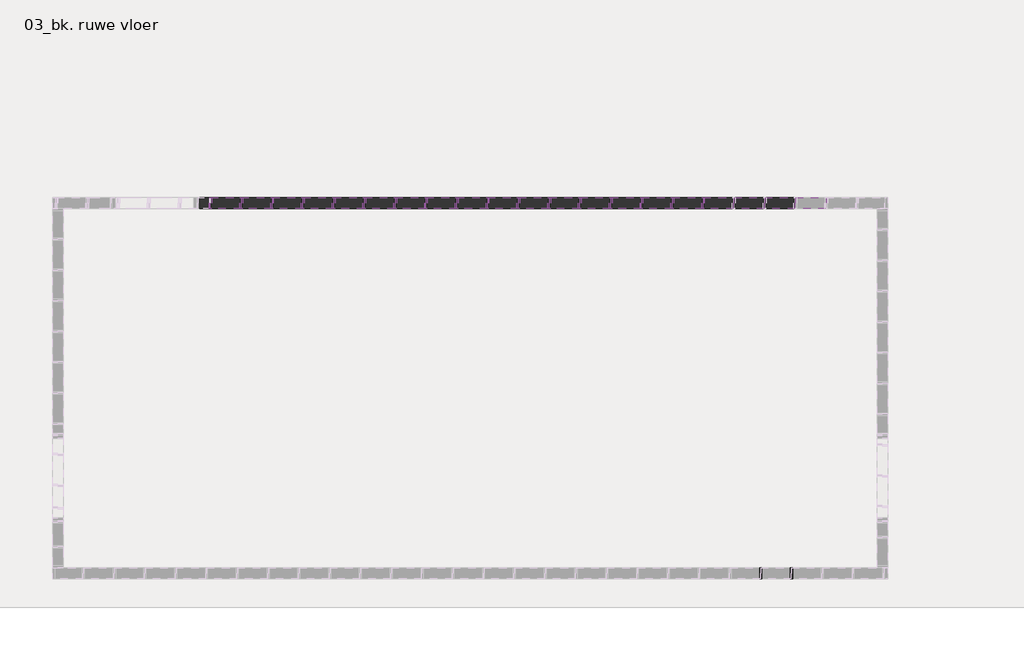
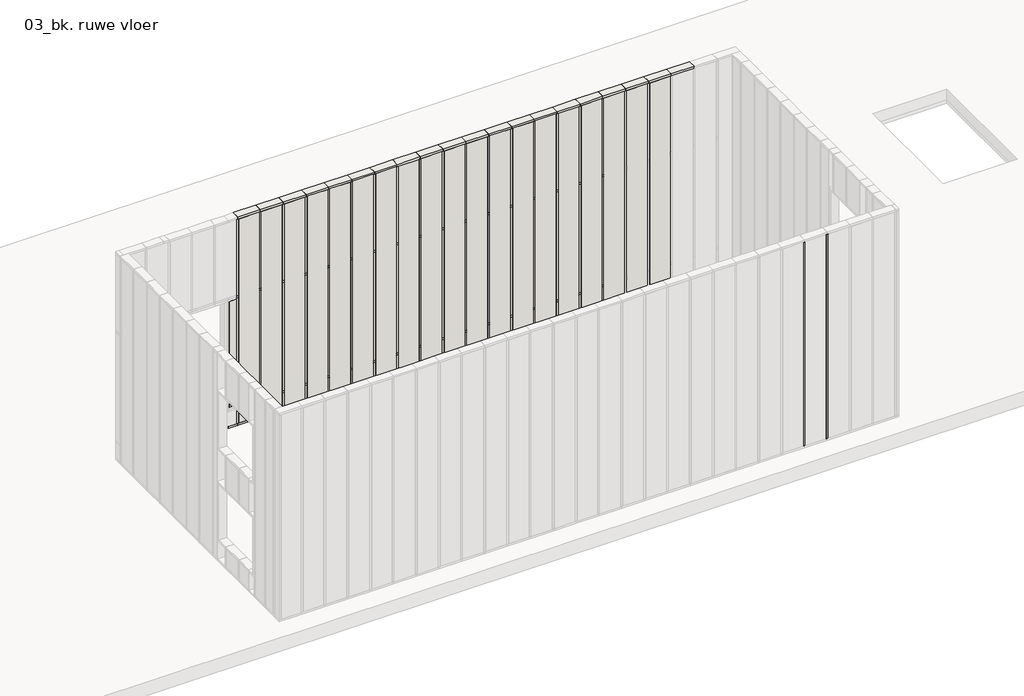
# One storey, part 3 of 9: 144 walls.
"""IFC4 building model written with IfcOpenShell, lengths in millimetres."""

import ifcopenshell
import ifcopenshell.guid

model = None  # the IFC model being written
_history = None  # IfcOwnerHistory: only IFC2X3 demands one
_inside = {}  # id of a spatial element -> (the spatial element, [elements in it])
_under = {}  # id of a project, library or spatial element -> (it, [spatial elements below it])
_declared = {}  # id of a project -> (the project, [libraries it declares])
_typed = {}  # id of a type object -> (the type object, [elements of that type])
_made_of = {}  # id of a material, layer set ... -> (it, [elements and type objects made of it])


def new_model(schema):
    """Start an empty IFC model of exactly this schema.

    Asked for "IFC4X3", IfcOpenShell would pick the latest addendum, in which some entities
    have other attributes; the version numbers below select the first issue.
    IFC2X3 requires an IfcOwnerHistory on every rooted entity: one is made here for all.
    """
    global model, _history
    if schema == "IFC4X3":
        model = ifcopenshell.file(schema_version=(4, 3, 0, 0))
    else:
        model = ifcopenshell.file(schema=schema)
    _inside.clear()
    _under.clear()
    _declared.clear()
    _typed.clear()
    _made_of.clear()
    _history = None
    if model.schema == "IFC2X3":
        org = make("IfcOrganization", Name="unknown")
        user = make(
            "IfcPersonAndOrganization",
            ThePerson=make("IfcPerson", FamilyName="unknown"),
            TheOrganization=org,
        )
        app = make(
            "IfcApplication",
            ApplicationDeveloper=org,
            Version="unknown",
            ApplicationFullName="unknown",
            ApplicationIdentifier="unknown",
        )
        _history = make(
            "IfcOwnerHistory",
            OwningUser=user,
            OwningApplication=app,
            ChangeAction="ADDED",
            CreationDate=0,
        )
    return model


def make(cls, **values):
    """One entity of the class cls with the attributes given. An attribute that is None is left unset."""
    return model.create_entity(
        cls, **{name: value for name, value in values.items() if value is not None}
    )


def rooted(cls, **values):
    """An entity with a GlobalId (a new one), such as an element, a storey or a relation."""
    return make(cls, GlobalId=ifcopenshell.guid.new(), OwnerHistory=_history, **values)


def si_unit(unit_type, name, prefix=None):
    """IfcSIUnit, for example si_unit("LENGTHUNIT", "METRE", prefix="MILLI")."""
    return make("IfcSIUnit", UnitType=unit_type, Prefix=prefix, Name=name)


def assignment(units):
    """IfcUnitAssignment: the units of a project."""
    return None if units is None else make("IfcUnitAssignment", Units=units)


def point(xyz):
    """IfcCartesianPoint."""
    return None if xyz is None else make("IfcCartesianPoint", Coordinates=xyz)


def direction(xyz):
    """IfcDirection."""
    return None if xyz is None else make("IfcDirection", DirectionRatios=xyz)


def frame(location, z_axis=None, x_axis=None):
    """IfcAxis2Placement3D, a coordinate frame: its origin and axes. An axis left out is left unset."""
    return make(
        "IfcAxis2Placement3D",
        Location=point(location),
        Axis=direction(z_axis),
        RefDirection=direction(x_axis),
    )


def origin():
    """The frame at (0, 0, 0) with its axes left unset."""
    return frame((0.0, 0.0, 0.0))


def origin_with_axes():
    """The frame at (0, 0, 0) with the z axis (0, 0, 1) and the x axis (1, 0, 0) written out."""
    return frame((0.0, 0.0, 0.0), z_axis=(0.0, 0.0, 1.0), x_axis=(1.0, 0.0, 0.0))


def place(relative_to, where):
    """IfcLocalPlacement: puts the frame where relative to a parent placement (None: the world)."""
    return make(
        "IfcLocalPlacement", PlacementRelTo=relative_to, RelativePlacement=where
    )


def context(
    kind, dimensions, precision=None, world=None, true_north=None, identifier=None
):
    """IfcGeometricRepresentationContext, for example the 3D "Model" context."""
    return make(
        "IfcGeometricRepresentationContext",
        ContextIdentifier=identifier,
        ContextType=kind,
        CoordinateSpaceDimension=dimensions,
        Precision=precision,
        WorldCoordinateSystem=world,
        TrueNorth=true_north,
    )


def project(units=None, contexts=None):
    """IfcProject with its units and contexts."""
    return rooted(
        "IfcProject",
        Name="project",
        RepresentationContexts=contexts,
        UnitsInContext=assignment(units),
    )


def spatial(cls, under=None, at=None, **own):
    """A site, building, storey or space (cls), placed at a placement, below another one or the project."""
    s = rooted(cls, ObjectPlacement=at, **own)
    if under is not None:
        _under.setdefault(under.id(), (under, []))[1].append(s)
    return s


def polyline(points):
    """IfcPolyline through the points."""
    return make("IfcPolyline", Points=[point(p) for p in points])


def outline(outer, holes=None, kind="AREA"):
    """IfcArbitraryClosedProfileDef: a profile drawn as a closed curve; with holes, ...WithVoids."""
    if holes is None:
        return make("IfcArbitraryClosedProfileDef", ProfileType=kind, OuterCurve=outer)
    return make(
        "IfcArbitraryProfileDefWithVoids",
        ProfileType=kind,
        OuterCurve=outer,
        InnerCurves=holes,
    )


def extrude(swept, where, along, depth):
    """IfcExtrudedAreaSolid: the profile swept, set in the frame where, extruded along a direction by depth."""
    return make(
        "IfcExtrudedAreaSolid",
        SweptArea=swept,
        Position=where,
        ExtrudedDirection=direction(along),
        Depth=depth,
    )


def shape(context_of_items, identifier, shape_type, items):
    """IfcShapeRepresentation: the items that make up one representation, for example the "Body"."""
    return make(
        "IfcShapeRepresentation",
        ContextOfItems=context_of_items,
        RepresentationIdentifier=identifier,
        RepresentationType=shape_type,
        Items=items,
    )


def source(mapping_origin, context_of_items, identifier, shape_type, items):
    """IfcRepresentationMap: a shape defined once, which mapped items show again and again."""
    return make(
        "IfcRepresentationMap",
        MappingOrigin=mapping_origin,
        MappedRepresentation=shape(context_of_items, identifier, shape_type, items),
    )


def transform(
    local_origin,
    x_axis=None,
    y_axis=None,
    z_axis=None,
    scale=None,
    scale2=None,
    scale3=None,
    uniform=True,
):
    """IfcCartesianTransformationOperator3D, or its non-uniform kind. x_axis, y_axis, z_axis: its Axis1, 2, 3."""
    if uniform:
        return make(
            "IfcCartesianTransformationOperator3D",
            Axis1=direction(x_axis),
            Axis2=direction(y_axis),
            LocalOrigin=point(local_origin),
            Scale=scale,
            Axis3=direction(z_axis),
        )
    return make(
        "IfcCartesianTransformationOperator3DnonUniform",
        Axis1=direction(x_axis),
        Axis2=direction(y_axis),
        LocalOrigin=point(local_origin),
        Scale=scale,
        Axis3=direction(z_axis),
        Scale2=scale2,
        Scale3=scale3,
    )


def mapped(mapping_source, mapping_target):
    """IfcMappedItem: shows the shape of a source again, moved by a transform."""
    return make(
        "IfcMappedItem", MappingSource=mapping_source, MappingTarget=mapping_target
    )


def made_of(thing, what):
    """Note that an element or type object is made of a material, layer set ...; save() writes the relation."""
    if what is not None:
        _made_of.setdefault(what.id(), (what, []))[1].append(thing)
    return thing


def element(
    cls,
    number,
    at=None,
    inside=None,
    cuts=None,
    type_object=None,
    material=None,
    context=None,
    identifier="Body",
    shape_type=None,
    held_by="IfcProductDefinitionShape",
    body=None,
    shapes=None,
    **own,
):
    """One element of the class cls, such as IfcWall. Its Tag is "e" and its number.

    at: its placement. inside: the storey or other place that contains it. cuts: it is an
    opening in that element (IfcRelVoidsElement). A single representation is given by context,
    identifier, shape_type and body (its items); several are given by shapes. held_by: the class
    of the entity that holds the representations. save() writes the other relations.
    """
    e = rooted(cls, Tag="e%d" % number, ObjectPlacement=at, **own)
    if body is not None:
        shapes = [shape(context, identifier, shape_type, body)]
    if shapes is not None:
        e.Representation = make(held_by, Representations=shapes)
    if inside is not None:
        _inside.setdefault(inside.id(), (inside, []))[1].append(e)
    if cuts is not None:
        rooted(
            "IfcRelVoidsElement", RelatingBuildingElement=cuts, RelatedOpeningElement=e
        )
    if type_object is not None:
        _typed.setdefault(type_object.id(), (type_object, []))[1].append(e)
    return made_of(e, material)


def aggregate(whole, parts):
    """IfcRelAggregates: a whole, such as a stair, and the parts it consists of."""
    return rooted("IfcRelAggregates", RelatingObject=whole, RelatedObjects=parts)


def save(model, path):
    """Write the relations noted so far, then the file.

    IfcRelAggregates (storeys below a building ...), IfcRelContainedInSpatialStructure (elements
    in a storey), IfcRelDefinesByType, IfcRelAssociatesMaterial and IfcRelDeclares: one each for
    every whole, place, type object, material and project.
    """
    for whole, parts in _under.values():
        aggregate(whole, parts)
    for where, things in _inside.values():
        rooted(
            "IfcRelContainedInSpatialStructure",
            RelatedElements=things,
            RelatingStructure=where,
        )
    for kind, things in _typed.values():
        rooted("IfcRelDefinesByType", RelatedObjects=things, RelatingType=kind)
    for what, things in _made_of.values():
        rooted("IfcRelAssociatesMaterial", RelatedObjects=things, RelatingMaterial=what)
    for by, libraries in _declared.values():
        rooted("IfcRelDeclares", RelatingContext=by, RelatedDefinitions=libraries)
    model.write(path)


def rectangular_mullion_51268c3e(model_context):
    return source(origin(), model_context, "Body", "SweptSolid", [
        extrude(outline(polyline([(0.0, -71.0), (-38.0, -71.0), (-38.0, 71.0), (0.0, 71.0), (0.0, -71.0)])), frame((0.0, 0.0, -407.0), z_axis=(0.0, 0.0, 1.0), x_axis=(1.0, 0.0, 0.0)), (0.0, 0.0, 1.0), 407.0),
    ])


def rectangular_mullion_fd8aedfe(model_context):
    return source(origin(), model_context, "Body", "SweptSolid", [
        extrude(outline(polyline([(-38.0, -71.0), (-38.0, 71.0), (0.0, 71.0), (0.0, -71.0), (-38.0, -71.0)])), frame((0.0, 0.0, -407.0), z_axis=(0.0, 0.0, 1.0), x_axis=(1.0, 0.0, 0.0)), (0.0, 0.0, 1.0), 407.0),
    ])


def rectangular_mullion_bc699282(model_context):
    return source(origin(), model_context, "Body", "SweptSolid", [
        extrude(outline(polyline([(19.0, -71.0), (-19.0, -71.0), (-19.0, 71.0), (19.0, 71.0), (19.0, -71.0)])), frame((0.0, 0.0, -3849.0), z_axis=(0.0, 0.0, 1.0), x_axis=(1.0, 0.0, 0.0)), (0.0, 0.0, 1.0), 3849.0),
    ])


def rectangular_mullion_c53917db(model_context):
    return source(origin(), model_context, "Body", "SweptSolid", [
        extrude(outline(polyline([(19.0, -71.0), (-19.0, -71.0), (-19.0, 71.0), (19.0, 71.0), (19.0, -71.0)])), frame((0.0, 0.0, -295.0), z_axis=(0.0, 0.0, 1.0), x_axis=(1.0, 0.0, 0.0)), (0.0, 0.0, 1.0), 295.0),
    ])


def rectangular_mullion_c6f7c22d(model_context):
    return source(origin(), model_context, "Body", "SweptSolid", [
        extrude(outline(polyline([(-38.0, -71.0), (-38.0, 71.0), (0.0, 71.0), (0.0, -71.0), (-38.0, -71.0)])), frame((0.0, 0.0, -167.1558939), z_axis=(0.0, 0.0, 1.0), x_axis=(1.0, 0.0, 0.0)), (0.0, 0.0, 1.0), 167.1558939),
    ])


def rectangular_mullion_878a7b4c(model_context):
    return source(origin(), model_context, "Body", "SweptSolid", [
        extrude(outline(polyline([(19.0, -71.0), (-19.0, -71.0), (-19.0, 71.0), (19.0, 71.0), (19.0, -71.0)])), frame((0.0, 0.0, -1440.0), z_axis=(0.0, 0.0, 1.0), x_axis=(1.0, 0.0, 0.0)), (0.0, 0.0, 1.0), 1440.0),
    ])


def rectangular_mullion_c09c4bb1(model_context):
    return source(origin(), model_context, "Body", "SweptSolid", [
        extrude(outline(polyline([(19.0, -71.0), (-19.0, -71.0), (-19.0, 71.0), (19.0, 71.0), (19.0, -71.0)])), frame((0.0, 0.0, -38.0), z_axis=(0.0, 0.0, 1.0), x_axis=(1.0, 0.0, 0.0)), (0.0, 0.0, 1.0), 38.0),
    ])


def rectangular_mullion_39366410(model_context):
    return source(origin(), model_context, "Body", "SweptSolid", [
        extrude(outline(polyline([(19.0, -71.0), (-19.0, -71.0), (-19.0, 71.0), (19.0, 71.0), (19.0, -71.0)])), frame((0.0, 0.0, -2038.0), z_axis=(0.0, 0.0, 1.0), x_axis=(1.0, 0.0, 0.0)), (0.0, 0.0, 1.0), 2038.0),
    ])


def system_panel_efc5a8ab(model_context):
    return source(origin(), model_context, "Body", "SweptSolid", [
        extrude(outline(polyline([(0.0, -184.5), (0.0, 184.5), (295.0, 184.5), (333.0, 184.5), (2371.0, 184.5), (2409.0, 184.5), (3849.0, 184.5), (3849.0, -184.5), (2409.0, -184.5), (2371.0, -184.5), (333.0, -184.5), (295.0, -184.5), (0.0, -184.5)])), frame((0.0, -71.0, 0.0), z_axis=(0.0, 1.0, 0.0), x_axis=(0.0, 0.0, 1.0)), (0.0, 0.0, 1.0), 142.0),
    ])


def system_panel_6860f7c2(model_context):
    return source(origin(), model_context, "Body", "SweptSolid", [
        extrude(outline(polyline([(64.577947, -71.0), (-64.577947, -71.0), (-64.577947, 71.0), (64.577947, 71.0), (64.577947, -71.0)])), origin_with_axes(), (0.0, 0.0, 1.0), 2000.0),
    ])


model = new_model("IFC4")

# Units and contexts
model_context = context("Model", 3, world=origin())
ifc_project = project(units=[si_unit("LENGTHUNIT", "METRE", prefix="MILLI")], contexts=[model_context])

# Site, building, storey
site = spatial("IfcSite", under=ifc_project)
building = spatial("IfcBuilding", under=site)
storey = spatial("IfcBuildingStorey", under=building, Name="03_bk. ruwe vloer", Elevation=11330.0)

# Walls
placement = place(None, origin())
rectangular_mullion_shape = rectangular_mullion_51268c3e(model_context)
element("IfcWall", 1, ObjectType="Rectangular Mullion", at=placement, inside=storey, context=model_context, shape_type="MappedRepresentation", body=[
    mapped(rectangular_mullion_shape, transform((63849.9999997, 5200.0, 15255.0), x_axis=(0.0, 0.0, 1.0), y_axis=(0.0, 1.0, 0.0), z_axis=(-1.0, 0.0, 0.0))),
])
element("IfcWall", 2, ObjectType="Rectangular Mullion", at=placement, inside=storey, context=model_context, shape_type="MappedRepresentation", body=[
    mapped(rectangular_mullion_shape, transform((63442.9999997, 5200.0, 15255.0), x_axis=(0.0, 0.0, 1.0), y_axis=(0.0, 1.0, 0.0), z_axis=(-1.0, 0.0, 0.0))),
])
element("IfcWall", 3, ObjectType="Rectangular Mullion", at=placement, inside=storey, context=model_context, shape_type="MappedRepresentation", body=[
    mapped(rectangular_mullion_shape, transform((63035.9999997, 5200.0, 15255.0), x_axis=(0.0, 0.0, 1.0), y_axis=(0.0, 1.0, 0.0), z_axis=(-1.0, 0.0, 0.0))),
])
element("IfcWall", 4, ObjectType="Rectangular Mullion", at=placement, inside=storey, context=model_context, shape_type="MappedRepresentation", body=[
    mapped(rectangular_mullion_shape, transform((62628.9999997, 5200.0, 15255.0), x_axis=(0.0, 0.0, 1.0), y_axis=(0.0, 1.0, 0.0), z_axis=(-1.0, 0.0, 0.0))),
])
element("IfcWall", 5, ObjectType="Rectangular Mullion", at=placement, inside=storey, context=model_context, shape_type="MappedRepresentation", body=[
    mapped(rectangular_mullion_shape, transform((62221.9999997, 5200.0, 15255.0), x_axis=(0.0, 0.0, 1.0), y_axis=(0.0, 1.0, 0.0), z_axis=(-1.0, 0.0, 0.0))),
])
element("IfcWall", 6, ObjectType="Rectangular Mullion", at=placement, inside=storey, context=model_context, shape_type="MappedRepresentation", body=[
    mapped(rectangular_mullion_shape, transform((61814.9999997, 5200.0, 15255.0), x_axis=(0.0, 0.0, 1.0), y_axis=(0.0, 1.0, 0.0), z_axis=(-1.0, 0.0, 0.0))),
])
element("IfcWall", 7, ObjectType="Rectangular Mullion", at=placement, inside=storey, context=model_context, shape_type="MappedRepresentation", body=[
    mapped(rectangular_mullion_shape, transform((61407.9999997, 5200.0, 15255.0), x_axis=(0.0, 0.0, 1.0), y_axis=(0.0, 1.0, 0.0), z_axis=(-1.0, 0.0, 0.0))),
])
element("IfcWall", 8, ObjectType="Rectangular Mullion", at=placement, inside=storey, context=model_context, shape_type="MappedRepresentation", body=[
    mapped(rectangular_mullion_shape, transform((61000.9999997, 5200.0, 15255.0), x_axis=(0.0, 0.0, 1.0), y_axis=(0.0, 1.0, 0.0), z_axis=(-1.0, 0.0, 0.0))),
])
element("IfcWall", 9, ObjectType="Rectangular Mullion", at=placement, inside=storey, context=model_context, shape_type="MappedRepresentation", body=[
    mapped(rectangular_mullion_shape, transform((60593.9999997, 5200.0, 15255.0), x_axis=(0.0, 0.0, 1.0), y_axis=(0.0, 1.0, 0.0), z_axis=(-1.0, 0.0, 0.0))),
])
element("IfcWall", 10, ObjectType="Rectangular Mullion", at=placement, inside=storey, context=model_context, shape_type="MappedRepresentation", body=[
    mapped(rectangular_mullion_shape, transform((60186.9999997, 5200.0, 15255.0), x_axis=(0.0, 0.0, 1.0), y_axis=(0.0, 1.0, 0.0), z_axis=(-1.0, 0.0, 0.0))),
])
element("IfcWall", 11, ObjectType="Rectangular Mullion", at=placement, inside=storey, context=model_context, shape_type="MappedRepresentation", body=[
    mapped(rectangular_mullion_shape, transform((59779.9999997, 5200.0, 15255.0), x_axis=(0.0, 0.0, 1.0), y_axis=(0.0, 1.0, 0.0), z_axis=(-1.0, 0.0, 0.0))),
])
element("IfcWall", 12, ObjectType="Rectangular Mullion", at=placement, inside=storey, context=model_context, shape_type="MappedRepresentation", body=[
    mapped(rectangular_mullion_shape, transform((59372.9999997, 5200.0, 15255.0), x_axis=(0.0, 0.0, 1.0), y_axis=(0.0, 1.0, 0.0), z_axis=(-1.0, 0.0, 0.0))),
])
element("IfcWall", 13, ObjectType="Rectangular Mullion", at=placement, inside=storey, context=model_context, shape_type="MappedRepresentation", body=[
    mapped(rectangular_mullion_shape, transform((58965.9999997, 5200.0, 15255.0), x_axis=(0.0, 0.0, 1.0), y_axis=(0.0, 1.0, 0.0), z_axis=(-1.0, 0.0, 0.0))),
])
element("IfcWall", 14, ObjectType="Rectangular Mullion", at=placement, inside=storey, context=model_context, shape_type="MappedRepresentation", body=[
    mapped(rectangular_mullion_shape, transform((58558.9999997, 5200.0, 15255.0), x_axis=(0.0, 0.0, 1.0), y_axis=(0.0, 1.0, 0.0), z_axis=(-1.0, 0.0, 0.0))),
])
element("IfcWall", 15, ObjectType="Rectangular Mullion", at=placement, inside=storey, context=model_context, shape_type="MappedRepresentation", body=[
    mapped(rectangular_mullion_shape, transform((58151.9999997, 5200.0, 15255.0), x_axis=(0.0, 0.0, 1.0), y_axis=(0.0, 1.0, 0.0), z_axis=(-1.0, 0.0, 0.0))),
])
element("IfcWall", 16, ObjectType="Rectangular Mullion", at=placement, inside=storey, context=model_context, shape_type="MappedRepresentation", body=[
    mapped(rectangular_mullion_shape, transform((57744.9999997, 5200.0, 15255.0), x_axis=(0.0, 0.0, 1.0), y_axis=(0.0, 1.0, 0.0), z_axis=(-1.0, 0.0, 0.0))),
])
element("IfcWall", 17, ObjectType="Rectangular Mullion", at=placement, inside=storey, context=model_context, shape_type="MappedRepresentation", body=[
    mapped(rectangular_mullion_shape, transform((57337.9999997, 5200.0, 15255.0), x_axis=(0.0, 0.0, 1.0), y_axis=(0.0, 1.0, 0.0), z_axis=(-1.0, 0.0, 0.0))),
])
element("IfcWall", 18, ObjectType="Rectangular Mullion", at=placement, inside=storey, context=model_context, shape_type="MappedRepresentation", body=[
    mapped(rectangular_mullion_shape, transform((56930.9999997, 5200.0, 15255.0), x_axis=(0.0, 0.0, 1.0), y_axis=(0.0, 1.0, 0.0), z_axis=(-1.0, 0.0, 0.0))),
])
element("IfcWall", 19, ObjectType="Rectangular Mullion", at=placement, inside=storey, context=model_context, shape_type="MappedRepresentation", body=[
    mapped(rectangular_mullion_shape, transform((56523.9999997, 5200.0, 15255.0), x_axis=(0.0, 0.0, 1.0), y_axis=(0.0, 1.0, 0.0), z_axis=(-1.0, 0.0, 0.0))),
])
element("IfcWall", 20, ObjectType="Rectangular Mullion", at=placement, inside=storey, context=model_context, shape_type="MappedRepresentation", body=[
    mapped(rectangular_mullion_shape, transform((56116.9999997, 5200.0, 15255.0), x_axis=(0.0, 0.0, 1.0), y_axis=(0.0, 1.0, 0.0), z_axis=(-1.0, 0.0, 0.0))),
])
rectangular_mullion_2_shape = rectangular_mullion_fd8aedfe(model_context)
element("IfcWall", 21, ObjectType="Rectangular Mullion", at=placement, inside=storey, context=model_context, shape_type="MappedRepresentation", body=[
    mapped(rectangular_mullion_2_shape, transform((62628.9999997, 5200.0, 11330.0), x_axis=(0.0, 0.0, -1.0), y_axis=(0.0, 1.0, 0.0), z_axis=(1.0, 0.0, 0.0))),
])
element("IfcWall", 22, ObjectType="Rectangular Mullion", at=placement, inside=storey, context=model_context, shape_type="MappedRepresentation", body=[
    mapped(rectangular_mullion_2_shape, transform((62221.9999997, 5200.0, 11330.0), x_axis=(0.0, 0.0, -1.0), y_axis=(0.0, 1.0, 0.0), z_axis=(1.0, 0.0, 0.0))),
])
element("IfcWall", 23, ObjectType="Rectangular Mullion", at=placement, inside=storey, context=model_context, shape_type="MappedRepresentation", body=[
    mapped(rectangular_mullion_2_shape, transform((61814.9999997, 5200.0, 11330.0), x_axis=(0.0, 0.0, -1.0), y_axis=(0.0, 1.0, 0.0), z_axis=(1.0, 0.0, 0.0))),
])
element("IfcWall", 24, ObjectType="Rectangular Mullion", at=placement, inside=storey, context=model_context, shape_type="MappedRepresentation", body=[
    mapped(rectangular_mullion_2_shape, transform((61407.9999997, 5200.0, 11330.0), x_axis=(0.0, 0.0, -1.0), y_axis=(0.0, 1.0, 0.0), z_axis=(1.0, 0.0, 0.0))),
])
element("IfcWall", 25, ObjectType="Rectangular Mullion", at=placement, inside=storey, context=model_context, shape_type="MappedRepresentation", body=[
    mapped(rectangular_mullion_2_shape, transform((61000.9999997, 5200.0, 11330.0), x_axis=(0.0, 0.0, -1.0), y_axis=(0.0, 1.0, 0.0), z_axis=(1.0, 0.0, 0.0))),
])
element("IfcWall", 26, ObjectType="Rectangular Mullion", at=placement, inside=storey, context=model_context, shape_type="MappedRepresentation", body=[
    mapped(rectangular_mullion_2_shape, transform((60593.9999997, 5200.0, 11330.0), x_axis=(0.0, 0.0, -1.0), y_axis=(0.0, 1.0, 0.0), z_axis=(1.0, 0.0, 0.0))),
])
element("IfcWall", 27, ObjectType="Rectangular Mullion", at=placement, inside=storey, context=model_context, shape_type="MappedRepresentation", body=[
    mapped(rectangular_mullion_2_shape, transform((60186.9999997, 5200.0, 11330.0), x_axis=(0.0, 0.0, -1.0), y_axis=(0.0, 1.0, 0.0), z_axis=(1.0, 0.0, 0.0))),
])
element("IfcWall", 28, ObjectType="Rectangular Mullion", at=placement, inside=storey, context=model_context, shape_type="MappedRepresentation", body=[
    mapped(rectangular_mullion_2_shape, transform((59779.9999997, 5200.0, 11330.0), x_axis=(0.0, 0.0, -1.0), y_axis=(0.0, 1.0, 0.0), z_axis=(1.0, 0.0, 0.0))),
])
element("IfcWall", 29, ObjectType="Rectangular Mullion", at=placement, inside=storey, context=model_context, shape_type="MappedRepresentation", body=[
    mapped(rectangular_mullion_2_shape, transform((59372.9999997, 5200.0, 11330.0), x_axis=(0.0, 0.0, -1.0), y_axis=(0.0, 1.0, 0.0), z_axis=(1.0, 0.0, 0.0))),
])
element("IfcWall", 30, ObjectType="Rectangular Mullion", at=placement, inside=storey, context=model_context, shape_type="MappedRepresentation", body=[
    mapped(rectangular_mullion_2_shape, transform((58965.9999997, 5200.0, 11330.0), x_axis=(0.0, 0.0, -1.0), y_axis=(0.0, 1.0, 0.0), z_axis=(1.0, 0.0, 0.0))),
])
element("IfcWall", 31, ObjectType="Rectangular Mullion", at=placement, inside=storey, context=model_context, shape_type="MappedRepresentation", body=[
    mapped(rectangular_mullion_2_shape, transform((58558.9999997, 5200.0, 11330.0), x_axis=(0.0, 0.0, -1.0), y_axis=(0.0, 1.0, 0.0), z_axis=(1.0, 0.0, 0.0))),
])
element("IfcWall", 32, ObjectType="Rectangular Mullion", at=placement, inside=storey, context=model_context, shape_type="MappedRepresentation", body=[
    mapped(rectangular_mullion_2_shape, transform((58151.9999997, 5200.0, 11330.0), x_axis=(0.0, 0.0, -1.0), y_axis=(0.0, 1.0, 0.0), z_axis=(1.0, 0.0, 0.0))),
])
element("IfcWall", 33, ObjectType="Rectangular Mullion", at=placement, inside=storey, context=model_context, shape_type="MappedRepresentation", body=[
    mapped(rectangular_mullion_2_shape, transform((57744.9999997, 5200.0, 11330.0), x_axis=(0.0, 0.0, -1.0), y_axis=(0.0, 1.0, 0.0), z_axis=(1.0, 0.0, 0.0))),
])
element("IfcWall", 34, ObjectType="Rectangular Mullion", at=placement, inside=storey, context=model_context, shape_type="MappedRepresentation", body=[
    mapped(rectangular_mullion_2_shape, transform((57337.9999997, 5200.0, 11330.0), x_axis=(0.0, 0.0, -1.0), y_axis=(0.0, 1.0, 0.0), z_axis=(1.0, 0.0, 0.0))),
])
element("IfcWall", 35, ObjectType="Rectangular Mullion", at=placement, inside=storey, context=model_context, shape_type="MappedRepresentation", body=[
    mapped(rectangular_mullion_2_shape, transform((56930.9999997, 5200.0, 11330.0), x_axis=(0.0, 0.0, -1.0), y_axis=(0.0, 1.0, 0.0), z_axis=(1.0, 0.0, 0.0))),
])
element("IfcWall", 36, ObjectType="Rectangular Mullion", at=placement, inside=storey, context=model_context, shape_type="MappedRepresentation", body=[
    mapped(rectangular_mullion_2_shape, transform((56523.9999997, 5200.0, 11330.0), x_axis=(0.0, 0.0, -1.0), y_axis=(0.0, 1.0, 0.0), z_axis=(1.0, 0.0, 0.0))),
])
rectangular_mullion_3_shape = rectangular_mullion_bc699282(model_context)
element("IfcWall", 37, ObjectType="Rectangular Mullion", at=placement, inside=storey, context=model_context, shape_type="MappedRepresentation", body=[
    mapped(rectangular_mullion_3_shape, transform((63390.0000003, 300.0, 11368.0), x_axis=(1.0, 0.0, 0.0), y_axis=(0.0, -1.0, 0.0), z_axis=(0.0, 0.0, -1.0))),
])
element("IfcWall", 38, ObjectType="Rectangular Mullion", at=placement, inside=storey, context=model_context, shape_type="MappedRepresentation", body=[
    mapped(rectangular_mullion_3_shape, transform((63797.0000003, 300.0, 11368.0), x_axis=(1.0, 0.0, 0.0), y_axis=(0.0, -1.0, 0.0), z_axis=(0.0, 0.0, -1.0))),
])
rectangular_mullion_4_shape = rectangular_mullion_c53917db(model_context)
element("IfcWall", 39, ObjectType="Rectangular Mullion", at=placement, inside=storey, context=model_context, shape_type="MappedRepresentation", body=[
    mapped(rectangular_mullion_4_shape, transform((62628.9999997, 5200.0, 11368.0), x_axis=(-1.0, 0.0, 0.0), y_axis=(0.0, 1.0, 0.0), z_axis=(0.0, 0.0, -1.0))),
])
element("IfcWall", 40, ObjectType="Rectangular Mullion", at=placement, inside=storey, context=model_context, shape_type="MappedRepresentation", body=[
    mapped(rectangular_mullion_4_shape, transform((62221.9999997, 5200.0, 11368.0), x_axis=(-1.0, 0.0, 0.0), y_axis=(0.0, 1.0, 0.0), z_axis=(0.0, 0.0, -1.0))),
])
element("IfcWall", 41, ObjectType="Rectangular Mullion", at=placement, inside=storey, context=model_context, shape_type="MappedRepresentation", body=[
    mapped(rectangular_mullion_4_shape, transform((61814.9999997, 5200.0, 11368.0), x_axis=(-1.0, 0.0, 0.0), y_axis=(0.0, 1.0, 0.0), z_axis=(0.0, 0.0, -1.0))),
])
element("IfcWall", 42, ObjectType="Rectangular Mullion", at=placement, inside=storey, context=model_context, shape_type="MappedRepresentation", body=[
    mapped(rectangular_mullion_4_shape, transform((61407.9999997, 5200.0, 11368.0), x_axis=(-1.0, 0.0, 0.0), y_axis=(0.0, 1.0, 0.0), z_axis=(0.0, 0.0, -1.0))),
])
element("IfcWall", 43, ObjectType="Rectangular Mullion", at=placement, inside=storey, context=model_context, shape_type="MappedRepresentation", body=[
    mapped(rectangular_mullion_4_shape, transform((61000.9999997, 5200.0, 11368.0), x_axis=(-1.0, 0.0, 0.0), y_axis=(0.0, 1.0, 0.0), z_axis=(0.0, 0.0, -1.0))),
])
element("IfcWall", 44, ObjectType="Rectangular Mullion", at=placement, inside=storey, context=model_context, shape_type="MappedRepresentation", body=[
    mapped(rectangular_mullion_4_shape, transform((60593.9999997, 5200.0, 11368.0), x_axis=(-1.0, 0.0, 0.0), y_axis=(0.0, 1.0, 0.0), z_axis=(0.0, 0.0, -1.0))),
])
element("IfcWall", 45, ObjectType="Rectangular Mullion", at=placement, inside=storey, context=model_context, shape_type="MappedRepresentation", body=[
    mapped(rectangular_mullion_4_shape, transform((60186.9999997, 5200.0, 11368.0), x_axis=(-1.0, 0.0, 0.0), y_axis=(0.0, 1.0, 0.0), z_axis=(0.0, 0.0, -1.0))),
])
element("IfcWall", 46, ObjectType="Rectangular Mullion", at=placement, inside=storey, context=model_context, shape_type="MappedRepresentation", body=[
    mapped(rectangular_mullion_4_shape, transform((59779.9999997, 5200.0, 11368.0), x_axis=(-1.0, 0.0, 0.0), y_axis=(0.0, 1.0, 0.0), z_axis=(0.0, 0.0, -1.0))),
])
element("IfcWall", 47, ObjectType="Rectangular Mullion", at=placement, inside=storey, context=model_context, shape_type="MappedRepresentation", body=[
    mapped(rectangular_mullion_4_shape, transform((59372.9999997, 5200.0, 11368.0), x_axis=(-1.0, 0.0, 0.0), y_axis=(0.0, 1.0, 0.0), z_axis=(0.0, 0.0, -1.0))),
])
element("IfcWall", 48, ObjectType="Rectangular Mullion", at=placement, inside=storey, context=model_context, shape_type="MappedRepresentation", body=[
    mapped(rectangular_mullion_4_shape, transform((58965.9999997, 5200.0, 11368.0), x_axis=(-1.0, 0.0, 0.0), y_axis=(0.0, 1.0, 0.0), z_axis=(0.0, 0.0, -1.0))),
])
element("IfcWall", 49, ObjectType="Rectangular Mullion", at=placement, inside=storey, context=model_context, shape_type="MappedRepresentation", body=[
    mapped(rectangular_mullion_4_shape, transform((58558.9999997, 5200.0, 11368.0), x_axis=(-1.0, 0.0, 0.0), y_axis=(0.0, 1.0, 0.0), z_axis=(0.0, 0.0, -1.0))),
])
element("IfcWall", 50, ObjectType="Rectangular Mullion", at=placement, inside=storey, context=model_context, shape_type="MappedRepresentation", body=[
    mapped(rectangular_mullion_4_shape, transform((58151.9999997, 5200.0, 11368.0), x_axis=(-1.0, 0.0, 0.0), y_axis=(0.0, 1.0, 0.0), z_axis=(0.0, 0.0, -1.0))),
])
element("IfcWall", 51, ObjectType="Rectangular Mullion", at=placement, inside=storey, context=model_context, shape_type="MappedRepresentation", body=[
    mapped(rectangular_mullion_4_shape, transform((57744.9999997, 5200.0, 11368.0), x_axis=(-1.0, 0.0, 0.0), y_axis=(0.0, 1.0, 0.0), z_axis=(0.0, 0.0, -1.0))),
])
element("IfcWall", 52, ObjectType="Rectangular Mullion", at=placement, inside=storey, context=model_context, shape_type="MappedRepresentation", body=[
    mapped(rectangular_mullion_4_shape, transform((57337.9999997, 5200.0, 11368.0), x_axis=(-1.0, 0.0, 0.0), y_axis=(0.0, 1.0, 0.0), z_axis=(0.0, 0.0, -1.0))),
])
element("IfcWall", 53, ObjectType="Rectangular Mullion", at=placement, inside=storey, context=model_context, shape_type="MappedRepresentation", body=[
    mapped(rectangular_mullion_4_shape, transform((56930.9999997, 5200.0, 11368.0), x_axis=(-1.0, 0.0, 0.0), y_axis=(0.0, 1.0, 0.0), z_axis=(0.0, 0.0, -1.0))),
])
element("IfcWall", 54, ObjectType="Rectangular Mullion", at=placement, inside=storey, context=model_context, shape_type="MappedRepresentation", body=[
    mapped(rectangular_mullion_4_shape, transform((56523.9999997, 5200.0, 11368.0), x_axis=(-1.0, 0.0, 0.0), y_axis=(0.0, 1.0, 0.0), z_axis=(0.0, 0.0, -1.0))),
])
element("IfcWall", 55, ObjectType="Rectangular Mullion", at=placement, inside=storey, context=model_context, shape_type="MappedRepresentation", body=[
    mapped(rectangular_mullion_4_shape, transform((56116.9999997, 5200.0, 11368.0), x_axis=(-1.0, 0.0, 0.0), y_axis=(0.0, 1.0, 0.0), z_axis=(0.0, 0.0, -1.0))),
])
rectangular_mullion_5_shape = rectangular_mullion_c6f7c22d(model_context)
element("IfcWall", 56, ObjectType="Rectangular Mullion", at=placement, inside=storey, context=model_context, shape_type="MappedRepresentation", body=[
    mapped(rectangular_mullion_5_shape, transform((56116.9999997, 5200.0, 11330.0), x_axis=(0.0, 0.0, -1.0), y_axis=(0.0, 1.0, 0.0), z_axis=(1.0, 0.0, 0.0))),
])
rectangular_mullion_6_shape = rectangular_mullion_878a7b4c(model_context)
element("IfcWall", 57, ObjectType="Rectangular Mullion", at=placement, inside=storey, context=model_context, shape_type="MappedRepresentation", body=[
    mapped(rectangular_mullion_6_shape, transform((62628.9999997, 5200.0, 13777.0), x_axis=(-1.0, 0.0, 0.0), y_axis=(0.0, 1.0, 0.0), z_axis=(0.0, 0.0, -1.0))),
])
element("IfcWall", 58, ObjectType="Rectangular Mullion", at=placement, inside=storey, context=model_context, shape_type="MappedRepresentation", body=[
    mapped(rectangular_mullion_6_shape, transform((62221.9999997, 5200.0, 13777.0), x_axis=(-1.0, 0.0, 0.0), y_axis=(0.0, 1.0, 0.0), z_axis=(0.0, 0.0, -1.0))),
])
element("IfcWall", 59, ObjectType="Rectangular Mullion", at=placement, inside=storey, context=model_context, shape_type="MappedRepresentation", body=[
    mapped(rectangular_mullion_6_shape, transform((61814.9999997, 5200.0, 13777.0), x_axis=(-1.0, 0.0, 0.0), y_axis=(0.0, 1.0, 0.0), z_axis=(0.0, 0.0, -1.0))),
])
element("IfcWall", 60, ObjectType="Rectangular Mullion", at=placement, inside=storey, context=model_context, shape_type="MappedRepresentation", body=[
    mapped(rectangular_mullion_6_shape, transform((61407.9999997, 5200.0, 13777.0), x_axis=(-1.0, 0.0, 0.0), y_axis=(0.0, 1.0, 0.0), z_axis=(0.0, 0.0, -1.0))),
])
element("IfcWall", 61, ObjectType="Rectangular Mullion", at=placement, inside=storey, context=model_context, shape_type="MappedRepresentation", body=[
    mapped(rectangular_mullion_6_shape, transform((61000.9999997, 5200.0, 13777.0), x_axis=(-1.0, 0.0, 0.0), y_axis=(0.0, 1.0, 0.0), z_axis=(0.0, 0.0, -1.0))),
])
element("IfcWall", 62, ObjectType="Rectangular Mullion", at=placement, inside=storey, context=model_context, shape_type="MappedRepresentation", body=[
    mapped(rectangular_mullion_6_shape, transform((60593.9999997, 5200.0, 13777.0), x_axis=(-1.0, 0.0, 0.0), y_axis=(0.0, 1.0, 0.0), z_axis=(0.0, 0.0, -1.0))),
])
element("IfcWall", 63, ObjectType="Rectangular Mullion", at=placement, inside=storey, context=model_context, shape_type="MappedRepresentation", body=[
    mapped(rectangular_mullion_6_shape, transform((60186.9999997, 5200.0, 13777.0), x_axis=(-1.0, 0.0, 0.0), y_axis=(0.0, 1.0, 0.0), z_axis=(0.0, 0.0, -1.0))),
])
element("IfcWall", 64, ObjectType="Rectangular Mullion", at=placement, inside=storey, context=model_context, shape_type="MappedRepresentation", body=[
    mapped(rectangular_mullion_6_shape, transform((59779.9999997, 5200.0, 13777.0), x_axis=(-1.0, 0.0, 0.0), y_axis=(0.0, 1.0, 0.0), z_axis=(0.0, 0.0, -1.0))),
])
element("IfcWall", 65, ObjectType="Rectangular Mullion", at=placement, inside=storey, context=model_context, shape_type="MappedRepresentation", body=[
    mapped(rectangular_mullion_6_shape, transform((59372.9999997, 5200.0, 13777.0), x_axis=(-1.0, 0.0, 0.0), y_axis=(0.0, 1.0, 0.0), z_axis=(0.0, 0.0, -1.0))),
])
element("IfcWall", 66, ObjectType="Rectangular Mullion", at=placement, inside=storey, context=model_context, shape_type="MappedRepresentation", body=[
    mapped(rectangular_mullion_6_shape, transform((58965.9999997, 5200.0, 13777.0), x_axis=(-1.0, 0.0, 0.0), y_axis=(0.0, 1.0, 0.0), z_axis=(0.0, 0.0, -1.0))),
])
element("IfcWall", 67, ObjectType="Rectangular Mullion", at=placement, inside=storey, context=model_context, shape_type="MappedRepresentation", body=[
    mapped(rectangular_mullion_6_shape, transform((58558.9999997, 5200.0, 13777.0), x_axis=(-1.0, 0.0, 0.0), y_axis=(0.0, 1.0, 0.0), z_axis=(0.0, 0.0, -1.0))),
])
element("IfcWall", 68, ObjectType="Rectangular Mullion", at=placement, inside=storey, context=model_context, shape_type="MappedRepresentation", body=[
    mapped(rectangular_mullion_6_shape, transform((58151.9999997, 5200.0, 13777.0), x_axis=(-1.0, 0.0, 0.0), y_axis=(0.0, 1.0, 0.0), z_axis=(0.0, 0.0, -1.0))),
])
element("IfcWall", 69, ObjectType="Rectangular Mullion", at=placement, inside=storey, context=model_context, shape_type="MappedRepresentation", body=[
    mapped(rectangular_mullion_6_shape, transform((57744.9999997, 5200.0, 13777.0), x_axis=(-1.0, 0.0, 0.0), y_axis=(0.0, 1.0, 0.0), z_axis=(0.0, 0.0, -1.0))),
])
element("IfcWall", 70, ObjectType="Rectangular Mullion", at=placement, inside=storey, context=model_context, shape_type="MappedRepresentation", body=[
    mapped(rectangular_mullion_6_shape, transform((57337.9999997, 5200.0, 13777.0), x_axis=(-1.0, 0.0, 0.0), y_axis=(0.0, 1.0, 0.0), z_axis=(0.0, 0.0, -1.0))),
])
element("IfcWall", 71, ObjectType="Rectangular Mullion", at=placement, inside=storey, context=model_context, shape_type="MappedRepresentation", body=[
    mapped(rectangular_mullion_6_shape, transform((56930.9999997, 5200.0, 13777.0), x_axis=(-1.0, 0.0, 0.0), y_axis=(0.0, 1.0, 0.0), z_axis=(0.0, 0.0, -1.0))),
])
element("IfcWall", 72, ObjectType="Rectangular Mullion", at=placement, inside=storey, context=model_context, shape_type="MappedRepresentation", body=[
    mapped(rectangular_mullion_6_shape, transform((56523.9999997, 5200.0, 13777.0), x_axis=(-1.0, 0.0, 0.0), y_axis=(0.0, 1.0, 0.0), z_axis=(0.0, 0.0, -1.0))),
])
element("IfcWall", 73, ObjectType="Rectangular Mullion", at=placement, inside=storey, context=model_context, shape_type="MappedRepresentation", body=[
    mapped(rectangular_mullion_6_shape, transform((56116.9999997, 5200.0, 13777.0), x_axis=(-1.0, 0.0, 0.0), y_axis=(0.0, 1.0, 0.0), z_axis=(0.0, 0.0, -1.0))),
])
rectangular_mullion_7_shape = rectangular_mullion_c09c4bb1(model_context)
element("IfcWall", 74, ObjectType="Rectangular Mullion", at=placement, inside=storey, context=model_context, shape_type="MappedRepresentation", body=[
    mapped(rectangular_mullion_7_shape, transform((62628.9999997, 5200.0, 13739.0), x_axis=(-1.0, 0.0, 0.0), y_axis=(0.0, 1.0, 0.0), z_axis=(0.0, 0.0, -1.0))),
])
element("IfcWall", 75, ObjectType="Rectangular Mullion", at=placement, inside=storey, context=model_context, shape_type="MappedRepresentation", body=[
    mapped(rectangular_mullion_7_shape, transform((62221.9999997, 5200.0, 13739.0), x_axis=(-1.0, 0.0, 0.0), y_axis=(0.0, 1.0, 0.0), z_axis=(0.0, 0.0, -1.0))),
])
element("IfcWall", 76, ObjectType="Rectangular Mullion", at=placement, inside=storey, context=model_context, shape_type="MappedRepresentation", body=[
    mapped(rectangular_mullion_7_shape, transform((61814.9999997, 5200.0, 13739.0), x_axis=(-1.0, 0.0, 0.0), y_axis=(0.0, 1.0, 0.0), z_axis=(0.0, 0.0, -1.0))),
])
element("IfcWall", 77, ObjectType="Rectangular Mullion", at=placement, inside=storey, context=model_context, shape_type="MappedRepresentation", body=[
    mapped(rectangular_mullion_7_shape, transform((61407.9999997, 5200.0, 13739.0), x_axis=(-1.0, 0.0, 0.0), y_axis=(0.0, 1.0, 0.0), z_axis=(0.0, 0.0, -1.0))),
])
element("IfcWall", 78, ObjectType="Rectangular Mullion", at=placement, inside=storey, context=model_context, shape_type="MappedRepresentation", body=[
    mapped(rectangular_mullion_7_shape, transform((61000.9999997, 5200.0, 13739.0), x_axis=(-1.0, 0.0, 0.0), y_axis=(0.0, 1.0, 0.0), z_axis=(0.0, 0.0, -1.0))),
])
element("IfcWall", 79, ObjectType="Rectangular Mullion", at=placement, inside=storey, context=model_context, shape_type="MappedRepresentation", body=[
    mapped(rectangular_mullion_7_shape, transform((60593.9999997, 5200.0, 13739.0), x_axis=(-1.0, 0.0, 0.0), y_axis=(0.0, 1.0, 0.0), z_axis=(0.0, 0.0, -1.0))),
])
element("IfcWall", 80, ObjectType="Rectangular Mullion", at=placement, inside=storey, context=model_context, shape_type="MappedRepresentation", body=[
    mapped(rectangular_mullion_7_shape, transform((60186.9999997, 5200.0, 13739.0), x_axis=(-1.0, 0.0, 0.0), y_axis=(0.0, 1.0, 0.0), z_axis=(0.0, 0.0, -1.0))),
])
element("IfcWall", 81, ObjectType="Rectangular Mullion", at=placement, inside=storey, context=model_context, shape_type="MappedRepresentation", body=[
    mapped(rectangular_mullion_7_shape, transform((59779.9999997, 5200.0, 13739.0), x_axis=(-1.0, 0.0, 0.0), y_axis=(0.0, 1.0, 0.0), z_axis=(0.0, 0.0, -1.0))),
])
element("IfcWall", 82, ObjectType="Rectangular Mullion", at=placement, inside=storey, context=model_context, shape_type="MappedRepresentation", body=[
    mapped(rectangular_mullion_7_shape, transform((59372.9999997, 5200.0, 13739.0), x_axis=(-1.0, 0.0, 0.0), y_axis=(0.0, 1.0, 0.0), z_axis=(0.0, 0.0, -1.0))),
])
element("IfcWall", 83, ObjectType="Rectangular Mullion", at=placement, inside=storey, context=model_context, shape_type="MappedRepresentation", body=[
    mapped(rectangular_mullion_7_shape, transform((58965.9999997, 5200.0, 13739.0), x_axis=(-1.0, 0.0, 0.0), y_axis=(0.0, 1.0, 0.0), z_axis=(0.0, 0.0, -1.0))),
])
element("IfcWall", 84, ObjectType="Rectangular Mullion", at=placement, inside=storey, context=model_context, shape_type="MappedRepresentation", body=[
    mapped(rectangular_mullion_7_shape, transform((58558.9999997, 5200.0, 13739.0), x_axis=(-1.0, 0.0, 0.0), y_axis=(0.0, 1.0, 0.0), z_axis=(0.0, 0.0, -1.0))),
])
element("IfcWall", 85, ObjectType="Rectangular Mullion", at=placement, inside=storey, context=model_context, shape_type="MappedRepresentation", body=[
    mapped(rectangular_mullion_7_shape, transform((58151.9999997, 5200.0, 13739.0), x_axis=(-1.0, 0.0, 0.0), y_axis=(0.0, 1.0, 0.0), z_axis=(0.0, 0.0, -1.0))),
])
element("IfcWall", 86, ObjectType="Rectangular Mullion", at=placement, inside=storey, context=model_context, shape_type="MappedRepresentation", body=[
    mapped(rectangular_mullion_7_shape, transform((57744.9999997, 5200.0, 13739.0), x_axis=(-1.0, 0.0, 0.0), y_axis=(0.0, 1.0, 0.0), z_axis=(0.0, 0.0, -1.0))),
])
element("IfcWall", 87, ObjectType="Rectangular Mullion", at=placement, inside=storey, context=model_context, shape_type="MappedRepresentation", body=[
    mapped(rectangular_mullion_7_shape, transform((57337.9999997, 5200.0, 13739.0), x_axis=(-1.0, 0.0, 0.0), y_axis=(0.0, 1.0, 0.0), z_axis=(0.0, 0.0, -1.0))),
])
element("IfcWall", 88, ObjectType="Rectangular Mullion", at=placement, inside=storey, context=model_context, shape_type="MappedRepresentation", body=[
    mapped(rectangular_mullion_7_shape, transform((56930.9999997, 5200.0, 13739.0), x_axis=(-1.0, 0.0, 0.0), y_axis=(0.0, 1.0, 0.0), z_axis=(0.0, 0.0, -1.0))),
])
element("IfcWall", 89, ObjectType="Rectangular Mullion", at=placement, inside=storey, context=model_context, shape_type="MappedRepresentation", body=[
    mapped(rectangular_mullion_7_shape, transform((56523.9999997, 5200.0, 13739.0), x_axis=(-1.0, 0.0, 0.0), y_axis=(0.0, 1.0, 0.0), z_axis=(0.0, 0.0, -1.0))),
])
element("IfcWall", 90, ObjectType="Rectangular Mullion", at=placement, inside=storey, context=model_context, shape_type="MappedRepresentation", body=[
    mapped(rectangular_mullion_7_shape, transform((62628.9999997, 5200.0, 11663.0), x_axis=(-1.0, 0.0, 0.0), y_axis=(0.0, 1.0, 0.0), z_axis=(0.0, 0.0, -1.0))),
])
element("IfcWall", 91, ObjectType="Rectangular Mullion", at=placement, inside=storey, context=model_context, shape_type="MappedRepresentation", body=[
    mapped(rectangular_mullion_7_shape, transform((62221.9999997, 5200.0, 11663.0), x_axis=(-1.0, 0.0, 0.0), y_axis=(0.0, 1.0, 0.0), z_axis=(0.0, 0.0, -1.0))),
])
element("IfcWall", 92, ObjectType="Rectangular Mullion", at=placement, inside=storey, context=model_context, shape_type="MappedRepresentation", body=[
    mapped(rectangular_mullion_7_shape, transform((61814.9999997, 5200.0, 11663.0), x_axis=(-1.0, 0.0, 0.0), y_axis=(0.0, 1.0, 0.0), z_axis=(0.0, 0.0, -1.0))),
])
element("IfcWall", 93, ObjectType="Rectangular Mullion", at=placement, inside=storey, context=model_context, shape_type="MappedRepresentation", body=[
    mapped(rectangular_mullion_7_shape, transform((61407.9999997, 5200.0, 11663.0), x_axis=(-1.0, 0.0, 0.0), y_axis=(0.0, 1.0, 0.0), z_axis=(0.0, 0.0, -1.0))),
])
element("IfcWall", 94, ObjectType="Rectangular Mullion", at=placement, inside=storey, context=model_context, shape_type="MappedRepresentation", body=[
    mapped(rectangular_mullion_7_shape, transform((61000.9999997, 5200.0, 11663.0), x_axis=(-1.0, 0.0, 0.0), y_axis=(0.0, 1.0, 0.0), z_axis=(0.0, 0.0, -1.0))),
])
element("IfcWall", 95, ObjectType="Rectangular Mullion", at=placement, inside=storey, context=model_context, shape_type="MappedRepresentation", body=[
    mapped(rectangular_mullion_7_shape, transform((60593.9999997, 5200.0, 11663.0), x_axis=(-1.0, 0.0, 0.0), y_axis=(0.0, 1.0, 0.0), z_axis=(0.0, 0.0, -1.0))),
])
element("IfcWall", 96, ObjectType="Rectangular Mullion", at=placement, inside=storey, context=model_context, shape_type="MappedRepresentation", body=[
    mapped(rectangular_mullion_7_shape, transform((60186.9999997, 5200.0, 11663.0), x_axis=(-1.0, 0.0, 0.0), y_axis=(0.0, 1.0, 0.0), z_axis=(0.0, 0.0, -1.0))),
])
element("IfcWall", 97, ObjectType="Rectangular Mullion", at=placement, inside=storey, context=model_context, shape_type="MappedRepresentation", body=[
    mapped(rectangular_mullion_7_shape, transform((59779.9999997, 5200.0, 11663.0), x_axis=(-1.0, 0.0, 0.0), y_axis=(0.0, 1.0, 0.0), z_axis=(0.0, 0.0, -1.0))),
])
element("IfcWall", 98, ObjectType="Rectangular Mullion", at=placement, inside=storey, context=model_context, shape_type="MappedRepresentation", body=[
    mapped(rectangular_mullion_7_shape, transform((59372.9999997, 5200.0, 11663.0), x_axis=(-1.0, 0.0, 0.0), y_axis=(0.0, 1.0, 0.0), z_axis=(0.0, 0.0, -1.0))),
])
element("IfcWall", 99, ObjectType="Rectangular Mullion", at=placement, inside=storey, context=model_context, shape_type="MappedRepresentation", body=[
    mapped(rectangular_mullion_7_shape, transform((58965.9999997, 5200.0, 11663.0), x_axis=(-1.0, 0.0, 0.0), y_axis=(0.0, 1.0, 0.0), z_axis=(0.0, 0.0, -1.0))),
])
element("IfcWall", 100, ObjectType="Rectangular Mullion", at=placement, inside=storey, context=model_context, shape_type="MappedRepresentation", body=[
    mapped(rectangular_mullion_7_shape, transform((58558.9999997, 5200.0, 11663.0), x_axis=(-1.0, 0.0, 0.0), y_axis=(0.0, 1.0, 0.0), z_axis=(0.0, 0.0, -1.0))),
])
element("IfcWall", 101, ObjectType="Rectangular Mullion", at=placement, inside=storey, context=model_context, shape_type="MappedRepresentation", body=[
    mapped(rectangular_mullion_7_shape, transform((58151.9999997, 5200.0, 11663.0), x_axis=(-1.0, 0.0, 0.0), y_axis=(0.0, 1.0, 0.0), z_axis=(0.0, 0.0, -1.0))),
])
element("IfcWall", 102, ObjectType="Rectangular Mullion", at=placement, inside=storey, context=model_context, shape_type="MappedRepresentation", body=[
    mapped(rectangular_mullion_7_shape, transform((57744.9999997, 5200.0, 11663.0), x_axis=(-1.0, 0.0, 0.0), y_axis=(0.0, 1.0, 0.0), z_axis=(0.0, 0.0, -1.0))),
])
element("IfcWall", 103, ObjectType="Rectangular Mullion", at=placement, inside=storey, context=model_context, shape_type="MappedRepresentation", body=[
    mapped(rectangular_mullion_7_shape, transform((57337.9999997, 5200.0, 11663.0), x_axis=(-1.0, 0.0, 0.0), y_axis=(0.0, 1.0, 0.0), z_axis=(0.0, 0.0, -1.0))),
])
element("IfcWall", 104, ObjectType="Rectangular Mullion", at=placement, inside=storey, context=model_context, shape_type="MappedRepresentation", body=[
    mapped(rectangular_mullion_7_shape, transform((56930.9999997, 5200.0, 11663.0), x_axis=(-1.0, 0.0, 0.0), y_axis=(0.0, 1.0, 0.0), z_axis=(0.0, 0.0, -1.0))),
])
element("IfcWall", 105, ObjectType="Rectangular Mullion", at=placement, inside=storey, context=model_context, shape_type="MappedRepresentation", body=[
    mapped(rectangular_mullion_7_shape, transform((56523.9999997, 5200.0, 11663.0), x_axis=(-1.0, 0.0, 0.0), y_axis=(0.0, 1.0, 0.0), z_axis=(0.0, 0.0, -1.0))),
])
element("IfcWall", 106, ObjectType="Rectangular Mullion", at=placement, inside=storey, context=model_context, shape_type="MappedRepresentation", body=[
    mapped(rectangular_mullion_7_shape, transform((56116.9999997, 5200.0, 13739.0), x_axis=(-1.0, 0.0, 0.0), y_axis=(0.0, 1.0, 0.0), z_axis=(0.0, 0.0, -1.0))),
])
element("IfcWall", 107, ObjectType="Rectangular Mullion", at=placement, inside=storey, context=model_context, shape_type="MappedRepresentation", body=[
    mapped(rectangular_mullion_7_shape, transform((56116.9999997, 5200.0, 11663.0), x_axis=(-1.0, 0.0, 0.0), y_axis=(0.0, 1.0, 0.0), z_axis=(0.0, 0.0, -1.0))),
])
rectangular_mullion_8_shape = rectangular_mullion_39366410(model_context)
element("IfcWall", 108, ObjectType="Rectangular Mullion", at=placement, inside=storey, context=model_context, shape_type="MappedRepresentation", body=[
    mapped(rectangular_mullion_8_shape, transform((62628.9999997, 5200.0, 11701.0), x_axis=(-1.0, 0.0, 0.0), y_axis=(0.0, 1.0, 0.0), z_axis=(0.0, 0.0, -1.0))),
])
element("IfcWall", 109, ObjectType="Rectangular Mullion", at=placement, inside=storey, context=model_context, shape_type="MappedRepresentation", body=[
    mapped(rectangular_mullion_8_shape, transform((62221.9999997, 5200.0, 11701.0), x_axis=(-1.0, 0.0, 0.0), y_axis=(0.0, 1.0, 0.0), z_axis=(0.0, 0.0, -1.0))),
])
element("IfcWall", 110, ObjectType="Rectangular Mullion", at=placement, inside=storey, context=model_context, shape_type="MappedRepresentation", body=[
    mapped(rectangular_mullion_8_shape, transform((61814.9999997, 5200.0, 11701.0), x_axis=(-1.0, 0.0, 0.0), y_axis=(0.0, 1.0, 0.0), z_axis=(0.0, 0.0, -1.0))),
])
element("IfcWall", 111, ObjectType="Rectangular Mullion", at=placement, inside=storey, context=model_context, shape_type="MappedRepresentation", body=[
    mapped(rectangular_mullion_8_shape, transform((61407.9999997, 5200.0, 11701.0), x_axis=(-1.0, 0.0, 0.0), y_axis=(0.0, 1.0, 0.0), z_axis=(0.0, 0.0, -1.0))),
])
element("IfcWall", 112, ObjectType="Rectangular Mullion", at=placement, inside=storey, context=model_context, shape_type="MappedRepresentation", body=[
    mapped(rectangular_mullion_8_shape, transform((61000.9999997, 5200.0, 11701.0), x_axis=(-1.0, 0.0, 0.0), y_axis=(0.0, 1.0, 0.0), z_axis=(0.0, 0.0, -1.0))),
])
element("IfcWall", 113, ObjectType="Rectangular Mullion", at=placement, inside=storey, context=model_context, shape_type="MappedRepresentation", body=[
    mapped(rectangular_mullion_8_shape, transform((60593.9999997, 5200.0, 11701.0), x_axis=(-1.0, 0.0, 0.0), y_axis=(0.0, 1.0, 0.0), z_axis=(0.0, 0.0, -1.0))),
])
element("IfcWall", 114, ObjectType="Rectangular Mullion", at=placement, inside=storey, context=model_context, shape_type="MappedRepresentation", body=[
    mapped(rectangular_mullion_8_shape, transform((60186.9999997, 5200.0, 11701.0), x_axis=(-1.0, 0.0, 0.0), y_axis=(0.0, 1.0, 0.0), z_axis=(0.0, 0.0, -1.0))),
])
element("IfcWall", 115, ObjectType="Rectangular Mullion", at=placement, inside=storey, context=model_context, shape_type="MappedRepresentation", body=[
    mapped(rectangular_mullion_8_shape, transform((59779.9999997, 5200.0, 11701.0), x_axis=(-1.0, 0.0, 0.0), y_axis=(0.0, 1.0, 0.0), z_axis=(0.0, 0.0, -1.0))),
])
element("IfcWall", 116, ObjectType="Rectangular Mullion", at=placement, inside=storey, context=model_context, shape_type="MappedRepresentation", body=[
    mapped(rectangular_mullion_8_shape, transform((59372.9999997, 5200.0, 11701.0), x_axis=(-1.0, 0.0, 0.0), y_axis=(0.0, 1.0, 0.0), z_axis=(0.0, 0.0, -1.0))),
])
element("IfcWall", 117, ObjectType="Rectangular Mullion", at=placement, inside=storey, context=model_context, shape_type="MappedRepresentation", body=[
    mapped(rectangular_mullion_8_shape, transform((58965.9999997, 5200.0, 11701.0), x_axis=(-1.0, 0.0, 0.0), y_axis=(0.0, 1.0, 0.0), z_axis=(0.0, 0.0, -1.0))),
])
element("IfcWall", 118, ObjectType="Rectangular Mullion", at=placement, inside=storey, context=model_context, shape_type="MappedRepresentation", body=[
    mapped(rectangular_mullion_8_shape, transform((58558.9999997, 5200.0, 11701.0), x_axis=(-1.0, 0.0, 0.0), y_axis=(0.0, 1.0, 0.0), z_axis=(0.0, 0.0, -1.0))),
])
element("IfcWall", 119, ObjectType="Rectangular Mullion", at=placement, inside=storey, context=model_context, shape_type="MappedRepresentation", body=[
    mapped(rectangular_mullion_8_shape, transform((58151.9999997, 5200.0, 11701.0), x_axis=(-1.0, 0.0, 0.0), y_axis=(0.0, 1.0, 0.0), z_axis=(0.0, 0.0, -1.0))),
])
element("IfcWall", 120, ObjectType="Rectangular Mullion", at=placement, inside=storey, context=model_context, shape_type="MappedRepresentation", body=[
    mapped(rectangular_mullion_8_shape, transform((57744.9999997, 5200.0, 11701.0), x_axis=(-1.0, 0.0, 0.0), y_axis=(0.0, 1.0, 0.0), z_axis=(0.0, 0.0, -1.0))),
])
element("IfcWall", 121, ObjectType="Rectangular Mullion", at=placement, inside=storey, context=model_context, shape_type="MappedRepresentation", body=[
    mapped(rectangular_mullion_8_shape, transform((57337.9999997, 5200.0, 11701.0), x_axis=(-1.0, 0.0, 0.0), y_axis=(0.0, 1.0, 0.0), z_axis=(0.0, 0.0, -1.0))),
])
element("IfcWall", 122, ObjectType="Rectangular Mullion", at=placement, inside=storey, context=model_context, shape_type="MappedRepresentation", body=[
    mapped(rectangular_mullion_8_shape, transform((56930.9999997, 5200.0, 11701.0), x_axis=(-1.0, 0.0, 0.0), y_axis=(0.0, 1.0, 0.0), z_axis=(0.0, 0.0, -1.0))),
])
element("IfcWall", 123, ObjectType="Rectangular Mullion", at=placement, inside=storey, context=model_context, shape_type="MappedRepresentation", body=[
    mapped(rectangular_mullion_8_shape, transform((56523.9999997, 5200.0, 11701.0), x_axis=(-1.0, 0.0, 0.0), y_axis=(0.0, 1.0, 0.0), z_axis=(0.0, 0.0, -1.0))),
])
element("IfcWall", 124, ObjectType="Rectangular Mullion", at=placement, inside=storey, context=model_context, shape_type="MappedRepresentation", body=[
    mapped(rectangular_mullion_8_shape, transform((56116.9999997, 5200.0, 11701.0), x_axis=(-1.0, 0.0, 0.0), y_axis=(0.0, 1.0, 0.0), z_axis=(0.0, 0.0, -1.0))),
])
system_panel_shape = system_panel_efc5a8ab(model_context)
element("IfcWall", 125, ObjectType="System Panel", at=placement, inside=storey, context=model_context, shape_type="MappedRepresentation", body=[
    mapped(system_panel_shape, transform((63646.4999997, 5200.0, 11368.0), x_axis=(-1.0, 0.0, 0.0), y_axis=(0.0, -1.0, 0.0), z_axis=(0.0, 0.0, 1.0))),
])
element("IfcWall", 126, ObjectType="System Panel", at=placement, inside=storey, context=model_context, shape_type="MappedRepresentation", body=[
    mapped(system_panel_shape, transform((63239.4999997, 5200.0, 11368.0), x_axis=(-1.0, 0.0, 0.0), y_axis=(0.0, -1.0, 0.0), z_axis=(0.0, 0.0, 1.0))),
])
element("IfcWall", 127, ObjectType="System Panel", at=placement, inside=storey, context=model_context, shape_type="MappedRepresentation", body=[
    mapped(system_panel_shape, transform((62832.4999997, 5200.0, 11368.0), x_axis=(-1.0, 0.0, 0.0), y_axis=(0.0, -1.0, 0.0), z_axis=(0.0, 0.0, 1.0))),
])
element("IfcWall", 128, ObjectType="System Panel", at=placement, inside=storey, context=model_context, shape_type="MappedRepresentation", body=[
    mapped(system_panel_shape, transform((62425.4999997, 5200.0, 11368.0), x_axis=(-1.0, 0.0, 0.0), y_axis=(0.0, -1.0, 0.0), z_axis=(0.0, 0.0, 1.0))),
])
element("IfcWall", 129, ObjectType="System Panel", at=placement, inside=storey, context=model_context, shape_type="MappedRepresentation", body=[
    mapped(system_panel_shape, transform((62018.4999997, 5200.0, 11368.0), x_axis=(-1.0, 0.0, 0.0), y_axis=(0.0, -1.0, 0.0), z_axis=(0.0, 0.0, 1.0))),
])
element("IfcWall", 130, ObjectType="System Panel", at=placement, inside=storey, context=model_context, shape_type="MappedRepresentation", body=[
    mapped(system_panel_shape, transform((61611.4999997, 5200.0, 11368.0), x_axis=(-1.0, 0.0, 0.0), y_axis=(0.0, -1.0, 0.0), z_axis=(0.0, 0.0, 1.0))),
])
element("IfcWall", 131, ObjectType="System Panel", at=placement, inside=storey, context=model_context, shape_type="MappedRepresentation", body=[
    mapped(system_panel_shape, transform((61204.4999997, 5200.0, 11368.0), x_axis=(-1.0, 0.0, 0.0), y_axis=(0.0, -1.0, 0.0), z_axis=(0.0, 0.0, 1.0))),
])
element("IfcWall", 132, ObjectType="System Panel", at=placement, inside=storey, context=model_context, shape_type="MappedRepresentation", body=[
    mapped(system_panel_shape, transform((60797.4999997, 5200.0, 11368.0), x_axis=(-1.0, 0.0, 0.0), y_axis=(0.0, -1.0, 0.0), z_axis=(0.0, 0.0, 1.0))),
])
element("IfcWall", 133, ObjectType="System Panel", at=placement, inside=storey, context=model_context, shape_type="MappedRepresentation", body=[
    mapped(system_panel_shape, transform((60390.4999997, 5200.0, 11368.0), x_axis=(-1.0, 0.0, 0.0), y_axis=(0.0, -1.0, 0.0), z_axis=(0.0, 0.0, 1.0))),
])
element("IfcWall", 134, ObjectType="System Panel", at=placement, inside=storey, context=model_context, shape_type="MappedRepresentation", body=[
    mapped(system_panel_shape, transform((59983.4999997, 5200.0, 11368.0), x_axis=(-1.0, 0.0, 0.0), y_axis=(0.0, -1.0, 0.0), z_axis=(0.0, 0.0, 1.0))),
])
element("IfcWall", 135, ObjectType="System Panel", at=placement, inside=storey, context=model_context, shape_type="MappedRepresentation", body=[
    mapped(system_panel_shape, transform((59576.4999997, 5200.0, 11368.0), x_axis=(-1.0, 0.0, 0.0), y_axis=(0.0, -1.0, 0.0), z_axis=(0.0, 0.0, 1.0))),
])
element("IfcWall", 136, ObjectType="System Panel", at=placement, inside=storey, context=model_context, shape_type="MappedRepresentation", body=[
    mapped(system_panel_shape, transform((59169.4999997, 5200.0, 11368.0), x_axis=(-1.0, 0.0, 0.0), y_axis=(0.0, -1.0, 0.0), z_axis=(0.0, 0.0, 1.0))),
])
element("IfcWall", 137, ObjectType="System Panel", at=placement, inside=storey, context=model_context, shape_type="MappedRepresentation", body=[
    mapped(system_panel_shape, transform((58762.4999997, 5200.0, 11368.0), x_axis=(-1.0, 0.0, 0.0), y_axis=(0.0, -1.0, 0.0), z_axis=(0.0, 0.0, 1.0))),
])
element("IfcWall", 138, ObjectType="System Panel", at=placement, inside=storey, context=model_context, shape_type="MappedRepresentation", body=[
    mapped(system_panel_shape, transform((58355.4999997, 5200.0, 11368.0), x_axis=(-1.0, 0.0, 0.0), y_axis=(0.0, -1.0, 0.0), z_axis=(0.0, 0.0, 1.0))),
])
element("IfcWall", 139, ObjectType="System Panel", at=placement, inside=storey, context=model_context, shape_type="MappedRepresentation", body=[
    mapped(system_panel_shape, transform((57948.4999997, 5200.0, 11368.0), x_axis=(-1.0, 0.0, 0.0), y_axis=(0.0, -1.0, 0.0), z_axis=(0.0, 0.0, 1.0))),
])
element("IfcWall", 140, ObjectType="System Panel", at=placement, inside=storey, context=model_context, shape_type="MappedRepresentation", body=[
    mapped(system_panel_shape, transform((57541.4999997, 5200.0, 11368.0), x_axis=(-1.0, 0.0, 0.0), y_axis=(0.0, -1.0, 0.0), z_axis=(0.0, 0.0, 1.0))),
])
element("IfcWall", 141, ObjectType="System Panel", at=placement, inside=storey, context=model_context, shape_type="MappedRepresentation", body=[
    mapped(system_panel_shape, transform((57134.4999997, 5200.0, 11368.0), x_axis=(-1.0, 0.0, 0.0), y_axis=(0.0, -1.0, 0.0), z_axis=(0.0, 0.0, 1.0))),
])
element("IfcWall", 142, ObjectType="System Panel", at=placement, inside=storey, context=model_context, shape_type="MappedRepresentation", body=[
    mapped(system_panel_shape, transform((56727.4999997, 5200.0, 11368.0), x_axis=(-1.0, 0.0, 0.0), y_axis=(0.0, -1.0, 0.0), z_axis=(0.0, 0.0, 1.0))),
])
element("IfcWall", 143, ObjectType="System Panel", at=placement, inside=storey, context=model_context, shape_type="MappedRepresentation", body=[
    mapped(system_panel_shape, transform((56320.4999997, 5200.0, 11368.0), x_axis=(-1.0, 0.0, 0.0), y_axis=(0.0, -1.0, 0.0), z_axis=(0.0, 0.0, 1.0))),
])
system_panel_2_shape = system_panel_6860f7c2(model_context)
element("IfcWall", 144, ObjectType="System Panel", at=placement, inside=storey, context=model_context, shape_type="MappedRepresentation", body=[
    mapped(system_panel_2_shape, transform((56033.4220527, 5200.0, 11720.0), x_axis=(-1.0, 0.0, 0.0), y_axis=(0.0, -1.0, 0.0), z_axis=(0.0, 0.0, 1.0))),
])

save(model, "model.ifc")
